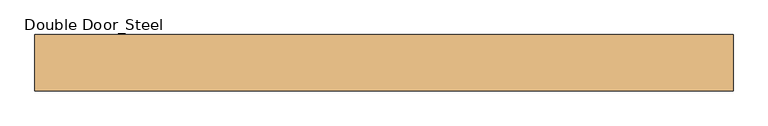
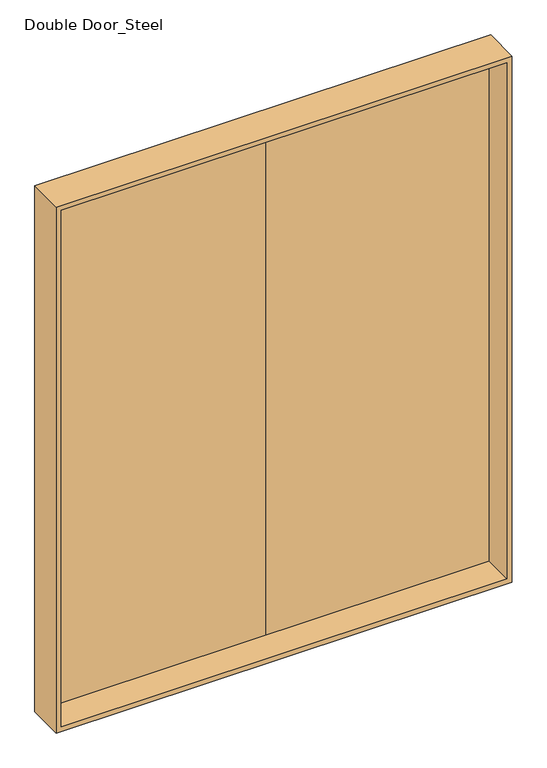
"""IFC4 building model written with IfcOpenShell, lengths in millimetres: door geometry, Double Door_Steel : H_DR_AR_B12_Double Door_Steel_W3100xH3780_FSD4."""

from ifc_helpers import new_model, si_unit, frame, origin, place, context, project, spatial, polyline, outline, extrude, faceted_brep, source, transform, mapped, element, save


def double_door_steel_fbc497f4(model_context):
    return source(origin(), model_context, "Body", "SolidModel", [
        extrude(outline(polyline([(1530.0, 85.0), (0.0, 85.0), (0.0, 125.0), (1530.0, 125.0), (1530.0, 85.0)])), frame((0.0, 0.0, 20.0), z_axis=(0.0, 0.0, 1.0), x_axis=(1.0, 0.0, 0.0)), (0.0, 0.0, 1.0), 3740.0),
        extrude(outline(polyline([(0.0, 85.0), (-1530.0, 85.0), (-1530.0, 125.0), (0.0, 125.0), (0.0, 85.0)])), frame((0.0, 0.0, 20.0), z_axis=(0.0, 0.0, 1.0), x_axis=(1.0, 0.0, 0.0)), (0.0, 0.0, 1.0), 3740.0),
        faceted_brep([(1550.0, -125.0, 3780.0), (1550.0, 125.0, 3780.0), (-1550.0, 125.0, 3780.0), (-1550.0, -125.0, 3780.0), (1515.0, 85.0, 3745.0), (1515.0, -125.0, 3745.0), (-1515.0, -125.0, 3745.0), (-1515.0, 85.0, 3745.0), (1530.0, 125.0, 3760.0), (1530.0, 85.0, 3760.0), (-1530.0, 85.0, 3760.0), (-1530.0, 125.0, 3760.0), (-1550.0, 125.0, 0.0), (-1550.0, -125.0, 0.0), (-1515.0, -125.0, 35.0), (-1515.0, 85.0, 35.0), (-1530.0, 85.0, 20.0), (-1530.0, 125.0, 20.0), (1550.0, 125.0, 0.0), (1530.0, 125.0, 20.0), (1550.0, -125.0, 0.0), (1515.0, -125.0, 35.0), (1515.0, 85.0, 35.0), (1530.0, 85.0, 20.0)], [[[0, 1, 2, 3]], [[4, 5, 6, 7]], [[8, 9, 10, 11]], [[3, 2, 12, 13]], [[7, 6, 14, 15]], [[11, 10, 16, 17]], [[18, 12, 2, 1], [8, 11, 17, 19]], [[13, 12, 18, 20]], [[0, 3, 13, 20], [21, 14, 6, 5]], [[15, 14, 21, 22]], [[23, 16, 10, 9], [4, 7, 15, 22]], [[17, 16, 23, 19]], [[20, 18, 1, 0]], [[22, 21, 5, 4]], [[19, 23, 9, 8]]]),
    ])


if __name__ == "__main__":
    model = new_model("IFC4")
    model_context = context("Model", 3, world=origin())
    ifc_project = project(units=[si_unit("LENGTHUNIT", "METRE", prefix="MILLI")], contexts=[model_context])
    site = spatial("IfcSite", under=ifc_project)
    building = spatial("IfcBuilding", under=site)
    placement = place(None, origin())
    double_door_steel_shape = double_door_steel_fbc497f4(model_context)
    element("IfcDoor", 1, ObjectType="Double Door_Steel : H_DR_AR_B12_Double Door_Steel_W3100xH3780_FSD4", at=placement, inside=building, context=model_context, shape_type="MappedRepresentation", body=[
        mapped(double_door_steel_shape, transform((0.0, 0.0, 0.0), x_axis=(1.0, 0.0, 0.0), y_axis=(0.0, 1.0, 0.0), z_axis=(0.0, 0.0, 1.0))),
    ])
    save(model, "model.ifc")

# Revit data of these elements
# Type "Double Door_Steel : H_DR_AR_B12_Double Door_Steel_W3100xH3780_FSD4"
#   Type Mark = "442"
#   프레임 = ""
#   철물 = ""
#   유리/마감 = ""
#   위치/개소 = ""
#   부호 = "1/SD"
#   문번호 = "4"
#   문기호 = "FSD"
#   Analytic Construction = "<None>"
#   Height = 3780 mm
#   Width = 3100 mm
#   Define Thermal Properties by = 1
#   문 틀 = none
#   문 = none
#   Function = (empty or 0)
#   Assembly Code = ""
#   Wall Closure = (empty or 0)
